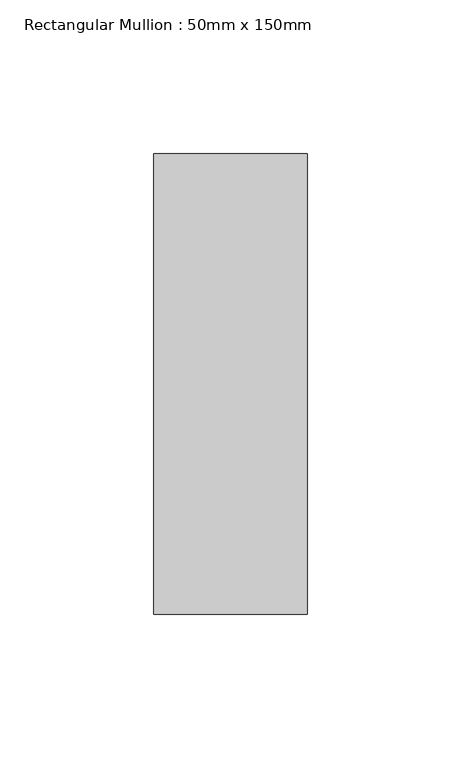
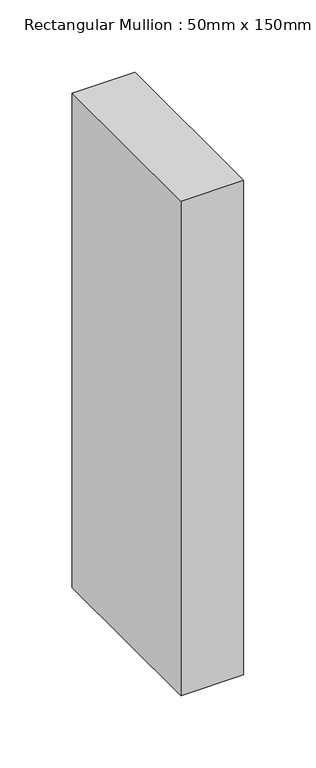
"""IFC4 building model written with IfcOpenShell, lengths in millimetres: member geometry, Rectangular Mullion : 50mm x 150mm."""

from ifc_helpers import new_model, si_unit, frame, origin, place, context, project, spatial, polyline, outline, extrude, source, transform, mapped, element, save


def rectangular_mullion_50mm_x_150mm_37616fee(model_context):
    return source(origin(), model_context, "Body", "SweptSolid", [
        extrude(outline(polyline([(0.0, 75.0), (0.0, -75.0), (-50.0, -75.0), (-50.0, 75.0), (0.0, 75.0)])), frame((0.0, 0.0, -416.6666667), z_axis=(0.0, 0.0, 1.0), x_axis=(1.0, 0.0, 0.0)), (0.0, 0.0, 1.0), 416.6666667),
    ])


if __name__ == "__main__":
    model = new_model("IFC4")
    model_context = context("Model", 3, world=origin())
    ifc_project = project(units=[si_unit("LENGTHUNIT", "METRE", prefix="MILLI")], contexts=[model_context])
    site = spatial("IfcSite", under=ifc_project)
    building = spatial("IfcBuilding", under=site)
    placement = place(None, origin())
    rectangular_mullion_50mm_x_150mm_shape = rectangular_mullion_50mm_x_150mm_37616fee(model_context)
    element("IfcMember", 1, ObjectType="Rectangular Mullion : 50mm x 150mm", at=placement, inside=building, context=model_context, shape_type="MappedRepresentation", body=[
        mapped(rectangular_mullion_50mm_x_150mm_shape, transform((0.0, 0.0, 0.0), x_axis=(1.0, 0.0, 0.0), y_axis=(0.0, 1.0, 0.0), z_axis=(0.0, 0.0, 1.0))),
    ])
    save(model, "model.ifc")

# Revit data of these elements
# Type "Rectangular Mullion : 50mm x 150mm"
#   built-in parameter 1007304 = 0.492126 (stored number, unit not read)
#   built-in parameter 1007301 = 0.082021 (stored number, unit not read)
#   built-in parameter 1007300 = 0.082021 (stored number, unit not read)
# Element 1 (IfcMember, "Rectangular Mullion : 50mm x 150mm")
#   Materials on its faces: "Aluminum"
# Materials
#   "Aluminum": class "Metal", colour RGB 244 244 244, transparency 0, Description = "Aluminum 6061", Cost = 0
